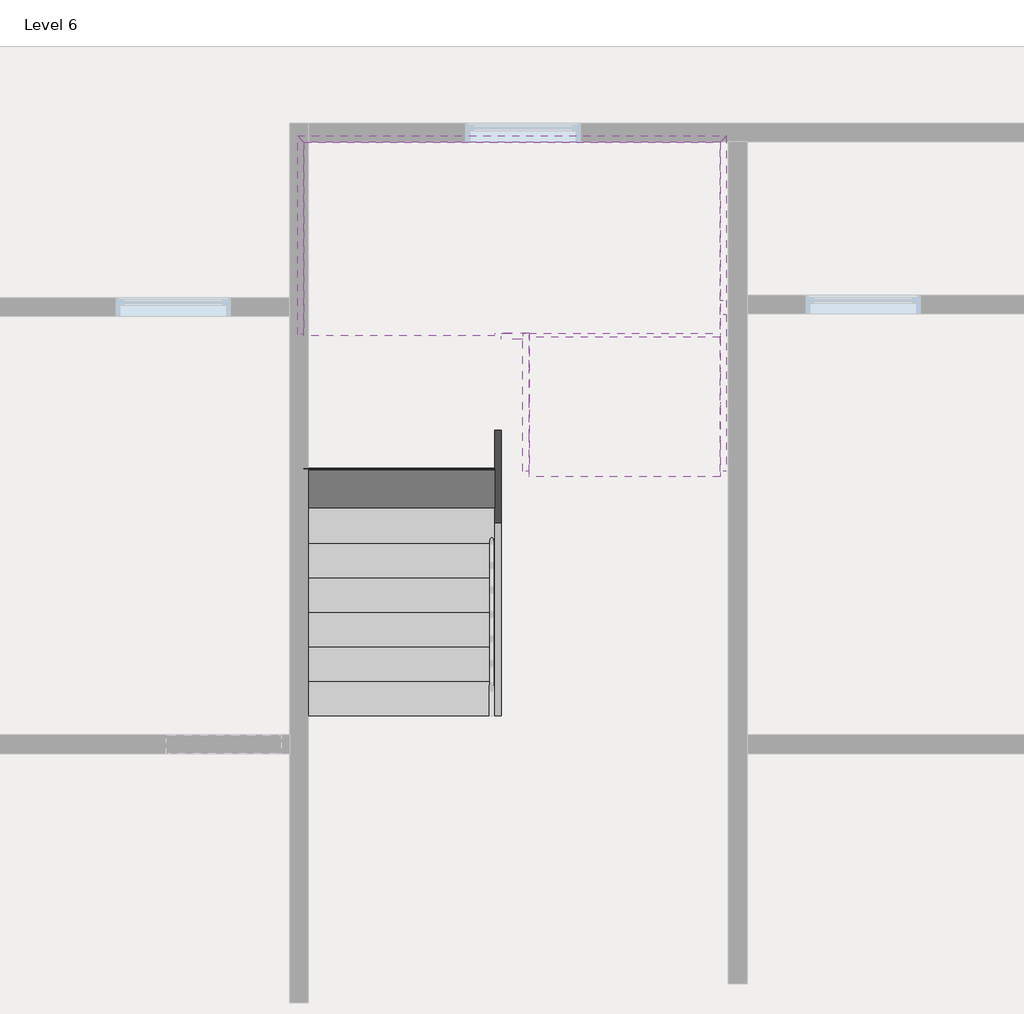
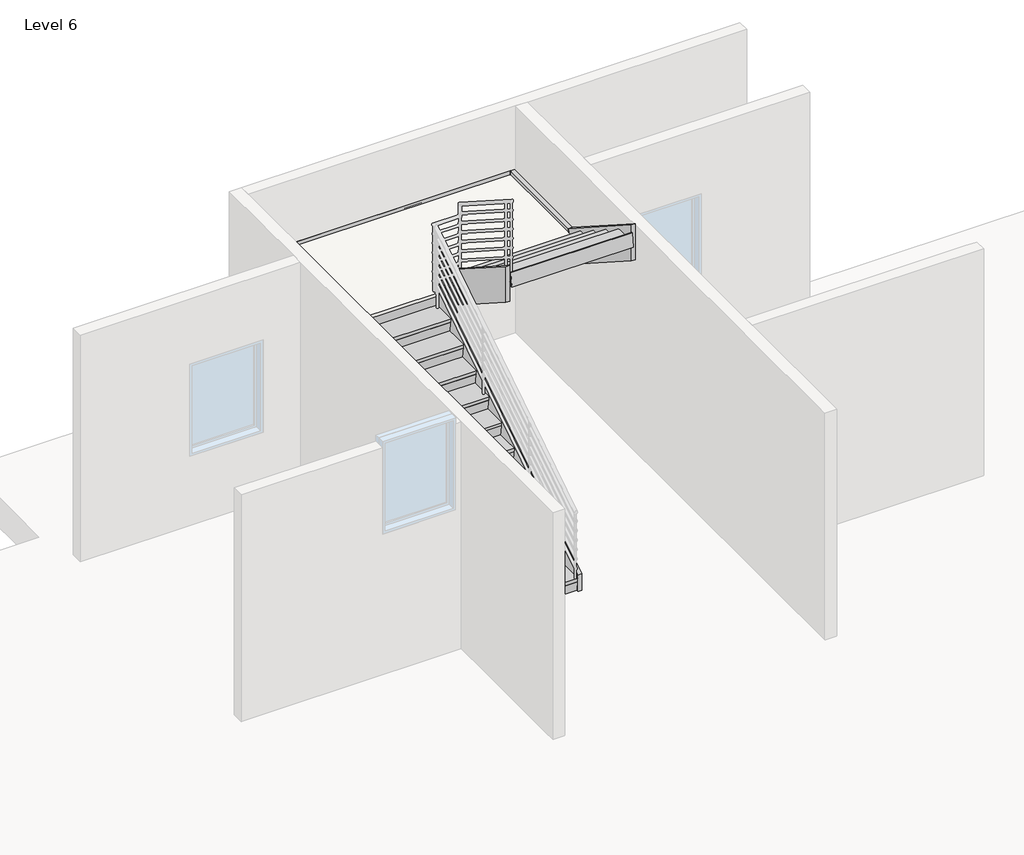
# One storey, part 7 of 7: 8 members, 2 stair flights, 1 slab.
"""IFC4 building model written with IfcOpenShell, lengths in millimetres."""

import ifcopenshell
import ifcopenshell.guid

model = None  # the IFC model being written
_history = None  # IfcOwnerHistory: only IFC2X3 demands one
_inside = {}  # id of a spatial element -> (the spatial element, [elements in it])
_under = {}  # id of a project, library or spatial element -> (it, [spatial elements below it])
_declared = {}  # id of a project -> (the project, [libraries it declares])
_typed = {}  # id of a type object -> (the type object, [elements of that type])
_made_of = {}  # id of a material, layer set ... -> (it, [elements and type objects made of it])


def new_model(schema):
    """Start an empty IFC model of exactly this schema.

    Asked for "IFC4X3", IfcOpenShell would pick the latest addendum, in which some entities
    have other attributes; the version numbers below select the first issue.
    IFC2X3 requires an IfcOwnerHistory on every rooted entity: one is made here for all.
    """
    global model, _history
    if schema == "IFC4X3":
        model = ifcopenshell.file(schema_version=(4, 3, 0, 0))
    else:
        model = ifcopenshell.file(schema=schema)
    _inside.clear()
    _under.clear()
    _declared.clear()
    _typed.clear()
    _made_of.clear()
    _history = None
    if model.schema == "IFC2X3":
        org = make("IfcOrganization", Name="unknown")
        user = make(
            "IfcPersonAndOrganization",
            ThePerson=make("IfcPerson", FamilyName="unknown"),
            TheOrganization=org,
        )
        app = make(
            "IfcApplication",
            ApplicationDeveloper=org,
            Version="unknown",
            ApplicationFullName="unknown",
            ApplicationIdentifier="unknown",
        )
        _history = make(
            "IfcOwnerHistory",
            OwningUser=user,
            OwningApplication=app,
            ChangeAction="ADDED",
            CreationDate=0,
        )
    return model


def make(cls, **values):
    """One entity of the class cls with the attributes given. An attribute that is None is left unset."""
    return model.create_entity(
        cls, **{name: value for name, value in values.items() if value is not None}
    )


def rooted(cls, **values):
    """An entity with a GlobalId (a new one), such as an element, a storey or a relation."""
    return make(cls, GlobalId=ifcopenshell.guid.new(), OwnerHistory=_history, **values)


def si_unit(unit_type, name, prefix=None):
    """IfcSIUnit, for example si_unit("LENGTHUNIT", "METRE", prefix="MILLI")."""
    return make("IfcSIUnit", UnitType=unit_type, Prefix=prefix, Name=name)


def assignment(units):
    """IfcUnitAssignment: the units of a project."""
    return None if units is None else make("IfcUnitAssignment", Units=units)


def point(xyz):
    """IfcCartesianPoint."""
    return None if xyz is None else make("IfcCartesianPoint", Coordinates=xyz)


def direction(xyz):
    """IfcDirection."""
    return None if xyz is None else make("IfcDirection", DirectionRatios=xyz)


def frame(location, z_axis=None, x_axis=None):
    """IfcAxis2Placement3D, a coordinate frame: its origin and axes. An axis left out is left unset."""
    return make(
        "IfcAxis2Placement3D",
        Location=point(location),
        Axis=direction(z_axis),
        RefDirection=direction(x_axis),
    )


def origin():
    """The frame at (0, 0, 0) with its axes left unset."""
    return frame((0.0, 0.0, 0.0))


def place(relative_to, where):
    """IfcLocalPlacement: puts the frame where relative to a parent placement (None: the world)."""
    return make(
        "IfcLocalPlacement", PlacementRelTo=relative_to, RelativePlacement=where
    )


def context(
    kind, dimensions, precision=None, world=None, true_north=None, identifier=None
):
    """IfcGeometricRepresentationContext, for example the 3D "Model" context."""
    return make(
        "IfcGeometricRepresentationContext",
        ContextIdentifier=identifier,
        ContextType=kind,
        CoordinateSpaceDimension=dimensions,
        Precision=precision,
        WorldCoordinateSystem=world,
        TrueNorth=true_north,
    )


def project(units=None, contexts=None):
    """IfcProject with its units and contexts."""
    return rooted(
        "IfcProject",
        Name="project",
        RepresentationContexts=contexts,
        UnitsInContext=assignment(units),
    )


def spatial(cls, under=None, at=None, **own):
    """A site, building, storey or space (cls), placed at a placement, below another one or the project."""
    s = rooted(cls, ObjectPlacement=at, **own)
    if under is not None:
        _under.setdefault(under.id(), (under, []))[1].append(s)
    return s


def polyline(points):
    """IfcPolyline through the points."""
    return make("IfcPolyline", Points=[point(p) for p in points])


def outline(outer, holes=None, kind="AREA"):
    """IfcArbitraryClosedProfileDef: a profile drawn as a closed curve; with holes, ...WithVoids."""
    if holes is None:
        return make("IfcArbitraryClosedProfileDef", ProfileType=kind, OuterCurve=outer)
    return make(
        "IfcArbitraryProfileDefWithVoids",
        ProfileType=kind,
        OuterCurve=outer,
        InnerCurves=holes,
    )


def extrude(swept, where, along, depth):
    """IfcExtrudedAreaSolid: the profile swept, set in the frame where, extruded along a direction by depth."""
    return make(
        "IfcExtrudedAreaSolid",
        SweptArea=swept,
        Position=where,
        ExtrudedDirection=direction(along),
        Depth=depth,
    )


def faces_of(points, faces, orient=None, outer=None):
    """IfcFace entities. A face is a list of loops; a loop is a list of indices into points, from 0.

    orient and outer hold one flag for each loop. By default every Orientation is true, the
    first loop of a face is its IfcFaceOuterBound and the others are IfcFaceBound.
    """
    made = []
    for i, loops in enumerate(faces):
        bounds = []
        for j, loop in enumerate(loops):
            is_outer = j == 0 if outer is None else outer[i][j]
            bounds.append(
                make(
                    "IfcFaceOuterBound" if is_outer else "IfcFaceBound",
                    Bound=make("IfcPolyLoop", Polygon=[points[k] for k in loop]),
                    Orientation=True if orient is None else orient[i][j],
                )
            )
        made.append(make("IfcFace", Bounds=bounds))
    return made


def faceted_brep(points, faces, orient=None, outer=None, voids=None):
    """IfcFacetedBrep: a solid bounded by flat faces; with voids (closed shells), ...WithVoids."""
    shared = [point(p) for p in points]
    hull = make("IfcClosedShell", CfsFaces=faces_of(shared, faces, orient, outer))
    if voids is None:
        return make("IfcFacetedBrep", Outer=hull)
    return make(
        "IfcFacetedBrepWithVoids",
        Outer=hull,
        Voids=[
            make(cls, CfsFaces=faces_of(shared, fs, o, b)) for cls, fs, o, b in voids
        ],
    )


def shape(context_of_items, identifier, shape_type, items):
    """IfcShapeRepresentation: the items that make up one representation, for example the "Body"."""
    return make(
        "IfcShapeRepresentation",
        ContextOfItems=context_of_items,
        RepresentationIdentifier=identifier,
        RepresentationType=shape_type,
        Items=items,
    )


def source(mapping_origin, context_of_items, identifier, shape_type, items):
    """IfcRepresentationMap: a shape defined once, which mapped items show again and again."""
    return make(
        "IfcRepresentationMap",
        MappingOrigin=mapping_origin,
        MappedRepresentation=shape(context_of_items, identifier, shape_type, items),
    )


def transform(
    local_origin,
    x_axis=None,
    y_axis=None,
    z_axis=None,
    scale=None,
    scale2=None,
    scale3=None,
    uniform=True,
):
    """IfcCartesianTransformationOperator3D, or its non-uniform kind. x_axis, y_axis, z_axis: its Axis1, 2, 3."""
    if uniform:
        return make(
            "IfcCartesianTransformationOperator3D",
            Axis1=direction(x_axis),
            Axis2=direction(y_axis),
            LocalOrigin=point(local_origin),
            Scale=scale,
            Axis3=direction(z_axis),
        )
    return make(
        "IfcCartesianTransformationOperator3DnonUniform",
        Axis1=direction(x_axis),
        Axis2=direction(y_axis),
        LocalOrigin=point(local_origin),
        Scale=scale,
        Axis3=direction(z_axis),
        Scale2=scale2,
        Scale3=scale3,
    )


def mapped(mapping_source, mapping_target):
    """IfcMappedItem: shows the shape of a source again, moved by a transform."""
    return make(
        "IfcMappedItem", MappingSource=mapping_source, MappingTarget=mapping_target
    )


def made_of(thing, what):
    """Note that an element or type object is made of a material, layer set ...; save() writes the relation."""
    if what is not None:
        _made_of.setdefault(what.id(), (what, []))[1].append(thing)
    return thing


def element(
    cls,
    number,
    at=None,
    inside=None,
    cuts=None,
    type_object=None,
    material=None,
    context=None,
    identifier="Body",
    shape_type=None,
    held_by="IfcProductDefinitionShape",
    body=None,
    shapes=None,
    **own,
):
    """One element of the class cls, such as IfcWall. Its Tag is "e" and its number.

    at: its placement. inside: the storey or other place that contains it. cuts: it is an
    opening in that element (IfcRelVoidsElement). A single representation is given by context,
    identifier, shape_type and body (its items); several are given by shapes. held_by: the class
    of the entity that holds the representations. save() writes the other relations.
    """
    e = rooted(cls, Tag="e%d" % number, ObjectPlacement=at, **own)
    if body is not None:
        shapes = [shape(context, identifier, shape_type, body)]
    if shapes is not None:
        e.Representation = make(held_by, Representations=shapes)
    if inside is not None:
        _inside.setdefault(inside.id(), (inside, []))[1].append(e)
    if cuts is not None:
        rooted(
            "IfcRelVoidsElement", RelatingBuildingElement=cuts, RelatedOpeningElement=e
        )
    if type_object is not None:
        _typed.setdefault(type_object.id(), (type_object, []))[1].append(e)
    return made_of(e, material)


def aggregate(whole, parts):
    """IfcRelAggregates: a whole, such as a stair, and the parts it consists of."""
    return rooted("IfcRelAggregates", RelatingObject=whole, RelatedObjects=parts)


def save(model, path):
    """Write the relations noted so far, then the file.

    IfcRelAggregates (storeys below a building ...), IfcRelContainedInSpatialStructure (elements
    in a storey), IfcRelDefinesByType, IfcRelAssociatesMaterial and IfcRelDeclares: one each for
    every whole, place, type object, material and project.
    """
    for whole, parts in _under.values():
        aggregate(whole, parts)
    for where, things in _inside.values():
        rooted(
            "IfcRelContainedInSpatialStructure",
            RelatedElements=things,
            RelatingStructure=where,
        )
    for kind, things in _typed.values():
        rooted("IfcRelDefinesByType", RelatedObjects=things, RelatingType=kind)
    for what, things in _made_of.values():
        rooted("IfcRelAssociatesMaterial", RelatedObjects=things, RelatingMaterial=what)
    for by, libraries in _declared.values():
        rooted("IfcRelDeclares", RelatingContext=by, RelatedDefinitions=libraries)
    model.write(path)


def non_monolithic_landing_c7120d81(model_context):
    return source(origin(), model_context, "Body", "Brep", [
        faceted_brep([(-226.7120949, 7307.4781803, 17617.6470588), (-226.7120949, 7300.3948469, 17567.6470588), (1293.2879051, 7300.3948469, 17567.6470588), (1293.2879051, 7307.4781803, 17617.6470588), (-499.4393676, 7309.7509075, 17617.6470588), (-499.4393676, 7332.4781803, 17617.6470588), (-226.7120949, 7332.4781803, 17617.6470588), (1293.2879051, 7332.4781803, 17617.6470588), (1293.2879051, 8852.4781803, 17617.6470588), (-2019.4393676, 8852.4781803, 17617.6470588), (-2019.4393676, 7309.7509075, 17617.6470588), (-226.7120949, 7332.4781803, 17567.6470588), (-499.4393676, 7332.4781803, 17567.6470588), (-499.4393676, 7316.8342409, 17567.6470588), (-2019.4393676, 7316.8342409, 17567.6470588), (-2019.4393676, 8852.4781803, 17567.6470588), (1293.2879051, 8852.4781803, 17567.6470588), (1293.2879051, 7332.4781803, 17567.6470588)], [[[0, 1, 2, 3]], [[4, 5, 6, 0, 3, 7, 8, 9, 10]], [[11, 12, 13, 14, 15, 16, 17, 2, 1]], [[5, 4, 13, 12]], [[6, 5, 12, 11]], [[0, 6, 11, 1]], [[7, 3, 2, 17]], [[8, 7, 17, 16]], [[9, 8, 16, 15]], [[10, 9, 15, 14]], [[4, 10, 14, 13]]]),
    ])


def stair_flight_50mm_tread_25mm_nosing_13mm_riser_3e0063ee(model_context):
    return source(origin(), model_context, "Body", "Brep", [
        faceted_brep([(-499.4393676, 4584.7509075, 15676.4705882), (-499.4393676, 4591.8342409, 15626.4705882), (-2019.4393676, 4591.8342409, 15626.4705882), (-2019.4393676, 4584.7509075, 15676.4705882), (-2019.4393676, 4284.7509075, 15676.4705882), (-499.4393676, 4284.7509075, 15676.4705882), (-499.4393676, 4291.8342409, 15626.4705882), (-2019.4393676, 4291.8342409, 15626.4705882)], [[[0, 1, 2, 3]], [[3, 4, 5, 0]], [[2, 1, 6, 7]], [[4, 3, 2, 7]], [[0, 5, 6, 1]], [[5, 4, 7, 6]]]),
        faceted_brep([(-499.4393676, 4291.8342409, 15626.4705882), (-499.4393676, 4309.7509075, 15500.0), (-499.4393676, 4322.3757185, 15500.0), (-499.4393676, 4304.4590518, 15626.4705882), (-2019.4393676, 4291.8342409, 15626.4705882), (-2019.4393676, 4304.4590518, 15626.4705882), (-2019.4393676, 4322.3757185, 15500.0), (-2019.4393676, 4309.7509075, 15500.0)], [[[0, 1, 2, 3]], [[4, 5, 6, 7]], [[1, 0, 4, 7]], [[2, 1, 7, 6]], [[3, 2, 6, 5]], [[0, 3, 5, 4]]]),
        faceted_brep([(-499.4393676, 4566.8342409, 15802.9411765), (-499.4393676, 4591.8342409, 15626.4705882), (-499.4393676, 4604.4590518, 15626.4705882), (-499.4393676, 4579.4590518, 15802.9411765), (-2019.4393676, 4566.8342409, 15802.9411765), (-2019.4393676, 4579.4590518, 15802.9411765), (-2019.4393676, 4604.4590518, 15626.4705882), (-2019.4393676, 4591.8342409, 15626.4705882)], [[[0, 1, 2, 3]], [[4, 5, 6, 7]], [[1, 0, 4, 7]], [[2, 1, 7, 6]], [[3, 2, 6, 5]], [[0, 3, 5, 4]]]),
        faceted_brep([(-2019.4393676, 4859.7509075, 15852.9411765), (-2019.4393676, 4559.7509075, 15852.9411765), (-499.4393676, 4559.7509075, 15852.9411765), (-499.4393676, 4859.7509075, 15852.9411765), (-2019.4393676, 4866.8342409, 15802.9411765), (-499.4393676, 4866.8342409, 15802.9411765), (-499.4393676, 4566.8342409, 15802.9411765), (-2019.4393676, 4566.8342409, 15802.9411765)], [[[0, 1, 2, 3]], [[4, 5, 6, 7]], [[1, 0, 4, 7]], [[3, 2, 6, 5]], [[3, 5, 4, 0]], [[2, 1, 7, 6]]]),
        faceted_brep([(-499.4393676, 4841.8342409, 15979.4117647), (-499.4393676, 4866.8342409, 15802.9411765), (-499.4393676, 4879.4590518, 15802.9411765), (-499.4393676, 4854.4590518, 15979.4117647), (-2019.4393676, 4841.8342409, 15979.4117647), (-2019.4393676, 4854.4590518, 15979.4117647), (-2019.4393676, 4879.4590518, 15802.9411765), (-2019.4393676, 4866.8342409, 15802.9411765)], [[[0, 1, 2, 3]], [[4, 5, 6, 7]], [[1, 0, 4, 7]], [[2, 1, 7, 6]], [[3, 2, 6, 5]], [[0, 3, 5, 4]]]),
        faceted_brep([(-2019.4393676, 5134.7509075, 16029.4117647), (-2019.4393676, 4834.7509075, 16029.4117647), (-499.4393676, 4834.7509075, 16029.4117647), (-499.4393676, 5134.7509075, 16029.4117647), (-2019.4393676, 5141.8342409, 15979.4117647), (-499.4393676, 5141.8342409, 15979.4117647), (-499.4393676, 4841.8342409, 15979.4117647), (-2019.4393676, 4841.8342409, 15979.4117647)], [[[0, 1, 2, 3]], [[4, 5, 6, 7]], [[1, 0, 4, 7]], [[3, 2, 6, 5]], [[3, 5, 4, 0]], [[2, 1, 7, 6]]]),
        faceted_brep([(-499.4393676, 5116.8342409, 16155.8823529), (-499.4393676, 5141.8342409, 15979.4117647), (-499.4393676, 5154.4590518, 15979.4117647), (-499.4393676, 5129.4590518, 16155.8823529), (-2019.4393676, 5116.8342409, 16155.8823529), (-2019.4393676, 5129.4590518, 16155.8823529), (-2019.4393676, 5154.4590518, 15979.4117647), (-2019.4393676, 5141.8342409, 15979.4117647)], [[[0, 1, 2, 3]], [[4, 5, 6, 7]], [[1, 0, 4, 7]], [[2, 1, 7, 6]], [[3, 2, 6, 5]], [[0, 3, 5, 4]]]),
        faceted_brep([(-2019.4393676, 5409.7509075, 16205.8823529), (-2019.4393676, 5109.7509075, 16205.8823529), (-499.4393676, 5109.7509075, 16205.8823529), (-499.4393676, 5409.7509075, 16205.8823529), (-2019.4393676, 5416.8342409, 16155.8823529), (-499.4393676, 5416.8342409, 16155.8823529), (-499.4393676, 5116.8342409, 16155.8823529), (-2019.4393676, 5116.8342409, 16155.8823529)], [[[0, 1, 2, 3]], [[4, 5, 6, 7]], [[1, 0, 4, 7]], [[3, 2, 6, 5]], [[3, 5, 4, 0]], [[2, 1, 7, 6]]]),
        faceted_brep([(-499.4393676, 5391.8342409, 16332.3529412), (-499.4393676, 5416.8342409, 16155.8823529), (-499.4393676, 5429.4590518, 16155.8823529), (-499.4393676, 5404.4590518, 16332.3529412), (-2019.4393676, 5391.8342409, 16332.3529412), (-2019.4393676, 5404.4590518, 16332.3529412), (-2019.4393676, 5429.4590518, 16155.8823529), (-2019.4393676, 5416.8342409, 16155.8823529)], [[[0, 1, 2, 3]], [[4, 5, 6, 7]], [[1, 0, 4, 7]], [[2, 1, 7, 6]], [[3, 2, 6, 5]], [[0, 3, 5, 4]]]),
        faceted_brep([(-2019.4393676, 5684.7509075, 16382.3529412), (-2019.4393676, 5384.7509075, 16382.3529412), (-499.4393676, 5384.7509075, 16382.3529412), (-499.4393676, 5684.7509075, 16382.3529412), (-2019.4393676, 5691.8342409, 16332.3529412), (-499.4393676, 5691.8342409, 16332.3529412), (-499.4393676, 5391.8342409, 16332.3529412), (-2019.4393676, 5391.8342409, 16332.3529412)], [[[0, 1, 2, 3]], [[4, 5, 6, 7]], [[1, 0, 4, 7]], [[3, 2, 6, 5]], [[3, 5, 4, 0]], [[2, 1, 7, 6]]]),
        faceted_brep([(-499.4393676, 5666.8342409, 16508.8235294), (-499.4393676, 5691.8342409, 16332.3529412), (-499.4393676, 5704.4590518, 16332.3529412), (-499.4393676, 5679.4590518, 16508.8235294), (-2019.4393676, 5666.8342409, 16508.8235294), (-2019.4393676, 5679.4590518, 16508.8235294), (-2019.4393676, 5704.4590518, 16332.3529412), (-2019.4393676, 5691.8342409, 16332.3529412)], [[[0, 1, 2, 3]], [[4, 5, 6, 7]], [[1, 0, 4, 7]], [[2, 1, 7, 6]], [[3, 2, 6, 5]], [[0, 3, 5, 4]]]),
        faceted_brep([(-2019.4393676, 5959.7509075, 16558.8235294), (-2019.4393676, 5659.7509075, 16558.8235294), (-499.4393676, 5659.7509075, 16558.8235294), (-499.4393676, 5959.7509075, 16558.8235294), (-2019.4393676, 5966.8342409, 16508.8235294), (-499.4393676, 5966.8342409, 16508.8235294), (-499.4393676, 5666.8342409, 16508.8235294), (-2019.4393676, 5666.8342409, 16508.8235294)], [[[0, 1, 2, 3]], [[4, 5, 6, 7]], [[1, 0, 4, 7]], [[3, 2, 6, 5]], [[3, 5, 4, 0]], [[2, 1, 7, 6]]]),
        faceted_brep([(-499.4393676, 5941.8342409, 16685.2941176), (-499.4393676, 5966.8342409, 16508.8235294), (-499.4393676, 5979.4590518, 16508.8235294), (-499.4393676, 5954.4590518, 16685.2941176), (-2019.4393676, 5941.8342409, 16685.2941176), (-2019.4393676, 5954.4590518, 16685.2941176), (-2019.4393676, 5979.4590518, 16508.8235294), (-2019.4393676, 5966.8342409, 16508.8235294)], [[[0, 1, 2, 3]], [[4, 5, 6, 7]], [[1, 0, 4, 7]], [[2, 1, 7, 6]], [[3, 2, 6, 5]], [[0, 3, 5, 4]]]),
        faceted_brep([(-2019.4393676, 6234.7509075, 16735.2941176), (-2019.4393676, 5934.7509075, 16735.2941176), (-499.4393676, 5934.7509075, 16735.2941176), (-499.4393676, 6234.7509075, 16735.2941176), (-2019.4393676, 6241.8342409, 16685.2941176), (-499.4393676, 6241.8342409, 16685.2941176), (-499.4393676, 5941.8342409, 16685.2941176), (-2019.4393676, 5941.8342409, 16685.2941176)], [[[0, 1, 2, 3]], [[4, 5, 6, 7]], [[1, 0, 4, 7]], [[3, 2, 6, 5]], [[3, 5, 4, 0]], [[2, 1, 7, 6]]]),
        faceted_brep([(-499.4393676, 6216.8342409, 16861.7647059), (-499.4393676, 6241.8342409, 16685.2941176), (-499.4393676, 6254.4590518, 16685.2941176), (-499.4393676, 6229.4590518, 16861.7647059), (-2019.4393676, 6216.8342409, 16861.7647059), (-2019.4393676, 6229.4590518, 16861.7647059), (-2019.4393676, 6254.4590518, 16685.2941176), (-2019.4393676, 6241.8342409, 16685.2941176)], [[[0, 1, 2, 3]], [[4, 5, 6, 7]], [[1, 0, 4, 7]], [[2, 1, 7, 6]], [[3, 2, 6, 5]], [[0, 3, 5, 4]]]),
        faceted_brep([(-2019.4393676, 6509.7509075, 16911.7647059), (-2019.4393676, 6209.7509075, 16911.7647059), (-499.4393676, 6209.7509075, 16911.7647059), (-499.4393676, 6509.7509075, 16911.7647059), (-2019.4393676, 6516.8342409, 16861.7647059), (-499.4393676, 6516.8342409, 16861.7647059), (-499.4393676, 6216.8342409, 16861.7647059), (-2019.4393676, 6216.8342409, 16861.7647059)], [[[0, 1, 2, 3]], [[4, 5, 6, 7]], [[1, 0, 4, 7]], [[3, 2, 6, 5]], [[3, 5, 4, 0]], [[2, 1, 7, 6]]]),
        faceted_brep([(-499.4393676, 6491.8342409, 17038.2352941), (-499.4393676, 6516.8342409, 16861.7647059), (-499.4393676, 6529.4590518, 16861.7647059), (-499.4393676, 6504.4590518, 17038.2352941), (-2019.4393676, 6491.8342409, 17038.2352941), (-2019.4393676, 6504.4590518, 17038.2352941), (-2019.4393676, 6529.4590518, 16861.7647059), (-2019.4393676, 6516.8342409, 16861.7647059)], [[[0, 1, 2, 3]], [[4, 5, 6, 7]], [[1, 0, 4, 7]], [[2, 1, 7, 6]], [[3, 2, 6, 5]], [[0, 3, 5, 4]]]),
        faceted_brep([(-2019.4393676, 6784.7509075, 17088.2352941), (-2019.4393676, 6484.7509075, 17088.2352941), (-499.4393676, 6484.7509075, 17088.2352941), (-499.4393676, 6784.7509075, 17088.2352941), (-2019.4393676, 6791.8342409, 17038.2352941), (-499.4393676, 6791.8342409, 17038.2352941), (-499.4393676, 6491.8342409, 17038.2352941), (-2019.4393676, 6491.8342409, 17038.2352941)], [[[0, 1, 2, 3]], [[4, 5, 6, 7]], [[1, 0, 4, 7]], [[3, 2, 6, 5]], [[3, 5, 4, 0]], [[2, 1, 7, 6]]]),
        faceted_brep([(-499.4393676, 6766.8342409, 17214.7058824), (-499.4393676, 6791.8342409, 17038.2352941), (-499.4393676, 6804.4590518, 17038.2352941), (-499.4393676, 6779.4590518, 17214.7058824), (-2019.4393676, 6766.8342409, 17214.7058824), (-2019.4393676, 6779.4590518, 17214.7058824), (-2019.4393676, 6804.4590518, 17038.2352941), (-2019.4393676, 6791.8342409, 17038.2352941)], [[[0, 1, 2, 3]], [[4, 5, 6, 7]], [[1, 0, 4, 7]], [[2, 1, 7, 6]], [[3, 2, 6, 5]], [[0, 3, 5, 4]]]),
        faceted_brep([(-2019.4393676, 7059.7509075, 17264.7058824), (-2019.4393676, 6759.7509075, 17264.7058824), (-499.4393676, 6759.7509075, 17264.7058824), (-499.4393676, 7059.7509075, 17264.7058824), (-2019.4393676, 7066.8342409, 17214.7058824), (-499.4393676, 7066.8342409, 17214.7058824), (-499.4393676, 6766.8342409, 17214.7058824), (-2019.4393676, 6766.8342409, 17214.7058824)], [[[0, 1, 2, 3]], [[4, 5, 6, 7]], [[1, 0, 4, 7]], [[3, 2, 6, 5]], [[3, 5, 4, 0]], [[2, 1, 7, 6]]]),
        faceted_brep([(-499.4393676, 7316.8342409, 17567.6470588), (-499.4393676, 7341.8342409, 17391.1764706), (-499.4393676, 7354.4590518, 17391.1764706), (-499.4393676, 7329.4590518, 17567.6470588), (-2019.4393676, 7316.8342409, 17567.6470588), (-2019.4393676, 7329.4590518, 17567.6470588), (-2019.4393676, 7354.4590518, 17391.1764706), (-2019.4393676, 7341.8342409, 17391.1764706)], [[[0, 1, 2, 3]], [[4, 5, 6, 7]], [[1, 0, 4, 7]], [[2, 1, 7, 6]], [[3, 2, 6, 5]], [[0, 3, 5, 4]]]),
        faceted_brep([(-499.4393676, 7041.8342409, 17391.1764706), (-499.4393676, 7066.8342409, 17214.7058824), (-499.4393676, 7079.4590518, 17214.7058824), (-499.4393676, 7054.4590518, 17391.1764706), (-2019.4393676, 7041.8342409, 17391.1764706), (-2019.4393676, 7054.4590518, 17391.1764706), (-2019.4393676, 7079.4590518, 17214.7058824), (-2019.4393676, 7066.8342409, 17214.7058824)], [[[0, 1, 2, 3]], [[4, 5, 6, 7]], [[1, 0, 4, 7]], [[2, 1, 7, 6]], [[3, 2, 6, 5]], [[0, 3, 5, 4]]]),
        faceted_brep([(-2019.4393676, 7334.7509075, 17441.1764706), (-2019.4393676, 7309.7509075, 17441.1764706), (-2019.4393676, 7034.7509075, 17441.1764706), (-499.4393676, 7034.7509075, 17441.1764706), (-499.4393676, 7334.7509075, 17441.1764706), (-2019.4393676, 7341.8342409, 17391.1764706), (-499.4393676, 7341.8342409, 17391.1764706), (-499.4393676, 7041.8342409, 17391.1764706), (-2019.4393676, 7041.8342409, 17391.1764706), (-2019.4393676, 7309.7509075, 17391.1764706)], [[[0, 1, 2, 3, 4]], [[5, 6, 7, 8, 9]], [[1, 0, 5, 9]], [[2, 1, 9, 8]], [[4, 3, 7, 6]], [[4, 6, 5, 0]], [[3, 2, 8, 7]]]),
    ])


def stair_flight_50mm_tread_25mm_nosing_13mm_riser_25054bb9(model_context):
    return source(origin(), model_context, "Body", "SweptSolid", [
        extrude(outline(polyline([(7032.4781803, 17794.1176471), (7332.4781803, 17794.1176471), (7325.3948469, 17744.1176471), (7025.3948469, 17744.1176471), (7032.4781803, 17794.1176471)])), frame((-226.7120949, 0.0, 0.0), z_axis=(1.0, 0.0, 0.0), x_axis=(0.0, 1.0, 0.0)), (0.0, 0.0, 1.0), 1520.0),
        extrude(outline(polyline([(7325.3948469, 17744.1176471), (7300.3948469, 17567.6470588), (7287.770036, 17567.6470588), (7312.770036, 17744.1176471), (7325.3948469, 17744.1176471)])), frame((-226.7120949, 0.0, 0.0), z_axis=(1.0, 0.0, 0.0), x_axis=(0.0, 1.0, 0.0)), (0.0, 0.0, 1.0), 1520.0),
        extrude(outline(polyline([(7050.3948469, 17920.5882353), (7025.3948469, 17744.1176471), (7012.770036, 17744.1176471), (7037.770036, 17920.5882353), (7050.3948469, 17920.5882353)])), frame((-226.7120949, 0.0, 0.0), z_axis=(1.0, 0.0, 0.0), x_axis=(0.0, 1.0, 0.0)), (0.0, 0.0, 1.0), 1520.0),
        extrude(outline(polyline([(6757.4781803, 17970.5882353), (7057.4781803, 17970.5882353), (7050.3948469, 17920.5882353), (6750.3948469, 17920.5882353), (6757.4781803, 17970.5882353)])), frame((-226.7120949, 0.0, 0.0), z_axis=(1.0, 0.0, 0.0), x_axis=(0.0, 1.0, 0.0)), (0.0, 0.0, 1.0), 1520.0),
        extrude(outline(polyline([(6775.3948469, 18097.0588235), (6750.3948469, 17920.5882353), (6737.770036, 17920.5882353), (6762.770036, 18097.0588235), (6775.3948469, 18097.0588235)])), frame((-226.7120949, 0.0, 0.0), z_axis=(1.0, 0.0, 0.0), x_axis=(0.0, 1.0, 0.0)), (0.0, 0.0, 1.0), 1520.0),
        extrude(outline(polyline([(6482.4781803, 18147.0588235), (6782.4781803, 18147.0588235), (6775.3948469, 18097.0588235), (6475.3948469, 18097.0588235), (6482.4781803, 18147.0588235)])), frame((-226.7120949, 0.0, 0.0), z_axis=(1.0, 0.0, 0.0), x_axis=(0.0, 1.0, 0.0)), (0.0, 0.0, 1.0), 1520.0),
        extrude(outline(polyline([(6500.3948469, 18273.5294118), (6475.3948469, 18097.0588235), (6462.770036, 18097.0588235), (6487.770036, 18273.5294118), (6500.3948469, 18273.5294118)])), frame((-226.7120949, 0.0, 0.0), z_axis=(1.0, 0.0, 0.0), x_axis=(0.0, 1.0, 0.0)), (0.0, 0.0, 1.0), 1520.0),
        extrude(outline(polyline([(6225.3948469, 18450.0), (6200.3948469, 18273.5294118), (6187.770036, 18273.5294118), (6212.770036, 18450.0), (6225.3948469, 18450.0)])), frame((-226.7120949, 0.0, 0.0), z_axis=(1.0, 0.0, 0.0), x_axis=(0.0, 1.0, 0.0)), (0.0, 0.0, 1.0), 1520.0),
        extrude(outline(polyline([(6207.4781803, 18323.5294118), (6507.4781803, 18323.5294118), (6500.3948469, 18273.5294118), (6200.3948469, 18273.5294118), (6207.4781803, 18323.5294118)])), frame((-226.7120949, 0.0, 0.0), z_axis=(1.0, 0.0, 0.0), x_axis=(0.0, 1.0, 0.0)), (0.0, 0.0, 1.0), 1520.0),
    ])


model = new_model("IFC4")

# Units and contexts
model_context = context("Model", 3, world=origin())
ifc_project = project(units=[si_unit("LENGTHUNIT", "METRE", prefix="MILLI")], contexts=[model_context])

# Site, building, storey
site = spatial("IfcSite", under=ifc_project)
building = spatial("IfcBuilding", under=site)
storey = spatial("IfcBuildingStorey", under=building, Name="Level 6", Elevation=15500.0)

# Members
placement = place(None, origin())
element("IfcMember", 1, ObjectType="Stringer - 50mm Width", at=placement, inside=storey, context=model_context, shape_type="SweptSolid", body=[
    extrude(outline(polyline([(4284.7509075, 15500.0), (4284.7509075, 15715.9811749), (7322.0354678, 17665.0407858), (7439.3399977, 17265.0407858), (4688.8181065, 15500.0), (4284.7509075, 15500.0)])), frame((-2069.4393676, 0.0, 0.0), z_axis=(1.0, 0.0, 0.0), x_axis=(0.0, 1.0, 0.0)), (0.0, 0.0, 1.0), 50.0),
])
element("IfcMember", 2, ObjectType="Stringer - 50mm Width", at=placement, inside=storey, context=model_context, shape_type="SweptSolid", body=[
    extrude(outline(polyline([(4284.7509075, 15500.0), (4284.7509075, 15715.9811749), (7322.0354678, 17665.0407858), (7332.4781803, 17665.0407858), (7332.4781803, 17196.4663575), (4688.8181065, 15500.0), (4284.7509075, 15500.0)])), frame((-499.4393676, 0.0, 0.0), z_axis=(1.0, 0.0, 0.0), x_axis=(0.0, 1.0, 0.0)), (0.0, 0.0, 1.0), 50.0),
])
element("IfcMember", 3, ObjectType="Stringer - 50mm Width", at=placement, inside=storey, context=model_context, shape_type="SweptSolid", body=[
    extrude(outline(polyline([(7595.19362, 17665.0407858), (7477.8890902, 17265.0407858), (6232.4781803, 18064.2349525), (6232.4781803, 18539.5105867), (7595.19362, 17665.0407858)])), frame((1293.2879051, 0.0, 0.0), z_axis=(1.0, 0.0, 0.0), x_axis=(0.0, 1.0, 0.0)), (0.0, 0.0, 1.0), 50.0),
])
element("IfcMember", 4, ObjectType="Stringer - 50mm Width", at=placement, inside=storey, context=model_context, shape_type="SweptSolid", body=[
    extrude(outline(polyline([(7332.4781803, 17833.6282338), (7332.4781803, 17358.3525996), (6232.4781803, 18064.2349525), (6232.4781803, 18539.5105867), (7332.4781803, 17833.6282338)])), frame((-276.7120949, 0.0, 0.0), z_axis=(1.0, 0.0, 0.0), x_axis=(0.0, 1.0, 0.0)), (0.0, 0.0, 1.0), 50.0),
])
element("IfcMember", 5, ObjectType="Stringer - 50mm Width", at=placement, inside=storey, context=model_context, shape_type="Brep", body=[
    faceted_brep([(1293.2879051, 7595.19362, 17665.0407858), (1343.2879051, 7595.19362, 17665.0407858), (1343.2879051, 8902.4781803, 17665.0407858), (1293.2879051, 8852.4781803, 17665.0407858), (1293.2879051, 7477.8890902, 17265.0407858), (1293.2879051, 8852.4781803, 17265.0407858), (1343.2879051, 7477.8890902, 17265.0407858), (1343.2879051, 8902.4781803, 17265.0407858)], [[[0, 1, 2, 3]], [[4, 0, 3, 5]], [[6, 4, 5, 7]], [[1, 6, 7, 2]], [[1, 0, 4, 6]], [[2, 7, 5, 3]]]),
])
element("IfcMember", 6, ObjectType="Stringer - 50mm Width", at=placement, inside=storey, context=model_context, shape_type="SweptSolid", body=[
    extrude(outline(polyline([(1343.2879051, 8902.4781803), (1293.2879051, 8852.4781803), (-2019.4393676, 8852.4781803), (-2069.4393676, 8902.4781803), (1343.2879051, 8902.4781803)])), frame((0.0, 0.0, 17265.0407858), z_axis=(0.0, 0.0, 1.0), x_axis=(1.0, 0.0, 0.0)), (0.0, 0.0, 1.0), 400.0),
])
element("IfcMember", 7, ObjectType="Stringer - 50mm Width", at=placement, inside=storey, context=model_context, shape_type="Brep", body=[
    faceted_brep([(-2019.4393676, 8852.4781803, 17665.0407858), (-2069.4393676, 8902.4781803, 17665.0407858), (-2069.4393676, 7322.0354678, 17665.0407858), (-2019.4393676, 7322.0354678, 17665.0407858), (-2019.4393676, 8852.4781803, 17265.0407858), (-2019.4393676, 7439.3399977, 17265.0407858), (-2069.4393676, 8902.4781803, 17265.0407858), (-2069.4393676, 7439.3399977, 17265.0407858)], [[[0, 1, 2, 3]], [[4, 0, 3, 5]], [[6, 4, 5, 7]], [[1, 6, 7, 2]], [[1, 0, 4, 6]], [[2, 7, 5, 3]]]),
])
element("IfcMember", 8, ObjectType="Stringer - 50mm Width", at=placement, inside=storey, context=model_context, shape_type="SweptSolid", body=[
    extrude(outline(polyline([(-449.4393676, 7282.4781803), (-449.4393676, 7332.4781803), (-276.7120949, 7332.4781803), (-276.7120949, 7282.4781803), (-449.4393676, 7282.4781803)])), frame((0.0, 0.0, 17265.0407858), z_axis=(0.0, 0.0, 1.0), x_axis=(1.0, 0.0, 0.0)), (0.0, 0.0, 1.0), 400.0),
])

# Slab
non_monolithic_landing_shape = non_monolithic_landing_c7120d81(model_context)
element("IfcSlab", 9, ObjectType="Non-Monolithic Landing", at=placement, inside=storey, context=model_context, shape_type="MappedRepresentation", body=[
    mapped(non_monolithic_landing_shape, transform((0.0, 0.0, 0.0), x_axis=(1.0, 0.0, 0.0), y_axis=(0.0, 1.0, 0.0), z_axis=(0.0, 0.0, 1.0))),
])

# Stair flights
stair_flight_50mm_tread_25mm_nosing_13mm_riser_shape = stair_flight_50mm_tread_25mm_nosing_13mm_riser_3e0063ee(model_context)
element("IfcStairFlight", 10, ObjectType="50mm Tread 25mm Nosing 13mm Riser", at=placement, inside=storey, context=model_context, shape_type="MappedRepresentation", body=[
    mapped(stair_flight_50mm_tread_25mm_nosing_13mm_riser_shape, transform((0.0, 0.0, 0.0), x_axis=(1.0, 0.0, 0.0), y_axis=(0.0, 1.0, 0.0), z_axis=(0.0, 0.0, 1.0))),
])
stair_flight_50mm_tread_25mm_nosing_13mm_riser_2_shape = stair_flight_50mm_tread_25mm_nosing_13mm_riser_25054bb9(model_context)
element("IfcStairFlight", 11, ObjectType="50mm Tread 25mm Nosing 13mm Riser", at=placement, inside=storey, context=model_context, shape_type="MappedRepresentation", body=[
    mapped(stair_flight_50mm_tread_25mm_nosing_13mm_riser_2_shape, transform((0.0, 0.0, 0.0), x_axis=(1.0, 0.0, 0.0), y_axis=(0.0, 1.0, 0.0), z_axis=(0.0, 0.0, 1.0))),
])

save(model, "model.ifc")

# Revit data of these elements
# Elements 1, 2, 3, 4, 5, 6, 7, 8 (IfcMember, "Stringer - 50mm Width")
#   Phase Created = New Construction
# Element 9 (IfcSlab, "Non-Monolithic Landing")
#   Phase Created = New Construction
# Elements 10, 11 (IfcStairFlight, "50mm Tread 25mm Nosing 13mm Riser")
#   Phase Created = New Construction
